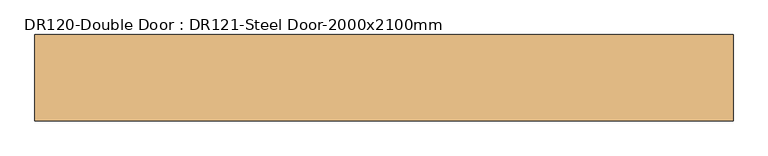
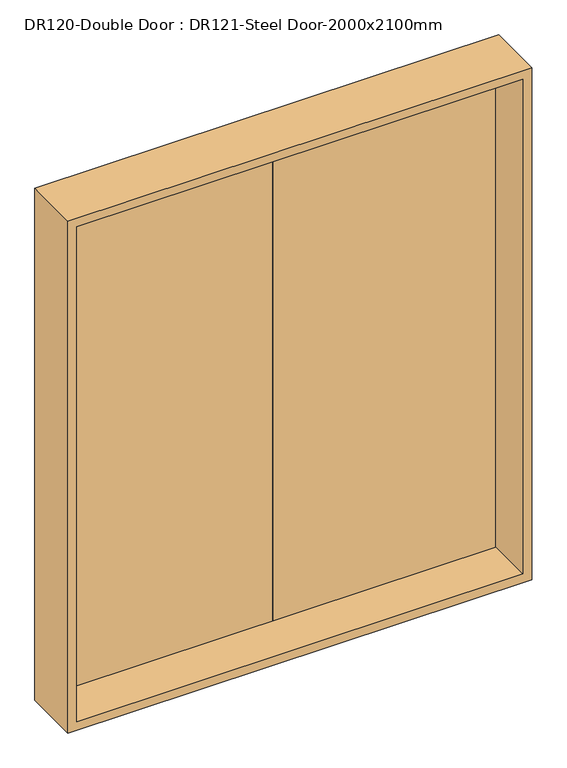
"""IFC4 building model written with IfcOpenShell, lengths in millimetres: door geometry, DR120-Double Door : DR121-Steel Door-2000x2100mm."""

from ifc_helpers import new_model, si_unit, frame, origin, place, context, project, spatial, polyline, outline, extrude, faceted_brep, source, transform, mapped, element, save


def dr120_double_door_dr121_steel_door_2000x2100mm_bb3c48ff(model_context):
    return source(origin(), model_context, "Body", "SolidModel", [
        extrude(outline(polyline([(880.0, 71.0), (0.0, 71.0), (0.0, 111.0), (880.0, 111.0), (880.0, 71.0)])), frame((0.0, 0.0, 20.0), z_axis=(0.0, 0.0, 1.0), x_axis=(1.0, 0.0, 0.0)), (0.0, 0.0, 1.0), 2060.0),
        extrude(outline(polyline([(0.0, 71.0), (-880.0, 71.0), (-880.0, 111.0), (0.0, 111.0), (0.0, 71.0)])), frame((0.0, 0.0, 20.0), z_axis=(0.0, 0.0, 1.0), x_axis=(1.0, 0.0, 0.0)), (0.0, 0.0, 1.0), 2060.0),
        faceted_brep([(900.0, -111.0, 2100.0), (900.0, 111.0, 2100.0), (-900.0, 111.0, 2100.0), (-900.0, -111.0, 2100.0), (865.0, 71.0, 2065.0), (865.0, -111.0, 2065.0), (-865.0, -111.0, 2065.0), (-865.0, 71.0, 2065.0), (880.0, 111.0, 2080.0), (880.0, 71.0, 2080.0), (-880.0, 71.0, 2080.0), (-880.0, 111.0, 2080.0), (-900.0, 111.0, 0.0), (-900.0, -111.0, 0.0), (-865.0, -111.0, 35.0), (-865.0, 71.0, 35.0), (-880.0, 71.0, 20.0), (-880.0, 111.0, 20.0), (900.0, 111.0, 0.0), (880.0, 111.0, 20.0), (900.0, -111.0, 0.0), (865.0, -111.0, 35.0), (865.0, 71.0, 35.0), (880.0, 71.0, 20.0)], [[[0, 1, 2, 3]], [[4, 5, 6, 7]], [[8, 9, 10, 11]], [[3, 2, 12, 13]], [[7, 6, 14, 15]], [[11, 10, 16, 17]], [[18, 12, 2, 1], [8, 11, 17, 19]], [[13, 12, 18, 20]], [[0, 3, 13, 20], [21, 14, 6, 5]], [[15, 14, 21, 22]], [[23, 16, 10, 9], [4, 7, 15, 22]], [[17, 16, 23, 19]], [[20, 18, 1, 0]], [[22, 21, 5, 4]], [[19, 23, 9, 8]]]),
    ])


if __name__ == "__main__":
    model = new_model("IFC4")
    model_context = context("Model", 3, world=origin())
    ifc_project = project(units=[si_unit("LENGTHUNIT", "METRE", prefix="MILLI")], contexts=[model_context])
    site = spatial("IfcSite", under=ifc_project)
    building = spatial("IfcBuilding", under=site)
    placement = place(None, origin())
    dr120_double_door_dr121_steel_door_2000x2100mm_shape = dr120_double_door_dr121_steel_door_2000x2100mm_bb3c48ff(model_context)
    element("IfcDoor", 1, ObjectType="DR120-Double Door : DR121-Steel Door-2000x2100mm", at=placement, inside=building, context=model_context, shape_type="MappedRepresentation", body=[
        mapped(dr120_double_door_dr121_steel_door_2000x2100mm_shape, transform((0.0, 0.0, 0.0), x_axis=(1.0, 0.0, 0.0), y_axis=(0.0, 1.0, 0.0), z_axis=(0.0, 0.0, 1.0))),
    ])
    save(model, "model.ifc")

# Revit data of these elements
# Type "DR120-Double Door : DR121-Steel Door-2000x2100mm"
#   Type Mark = "SD"
#   프레임 = ""
#   철물 = ""
#   유리/마감 = ""
#   위치/개소 = ""
#   부호 = "1/SD"
#   문번호 = ""
#   문기호 = "SD"
#   Analytic Construction = "<None>"
#   Height = 2100 mm
#   Width = 1800 mm
#   Define Thermal Properties by = 1
#   문 틀 = A04AQ098-00003_Steel Door_non FP_double
#   문 = 문
#   Function = (empty or 0)
#   Assembly Code = ""
#   Wall Closure = (empty or 0)
# Element 1 (IfcDoor, "DR120-Double Door : DR121-Steel Door-2000x2100mm")
#   Materials on its faces: "A04AQ098-00003_Steel Door_non FP_double", "문"
# Materials
#   "A04AQ098-00003_Steel Door_non FP_double": class "금속", colour RGB 247 247 247, transparency 0, Description = "Steel Door", W00) Work Master Code = "A04AQ098-00003", W01) Work Master_Lv1 = "Finishing Work", W02) Work Master_Lv2 = "Door & Window Work", W03) Work Master_Spec.1 = "Steel Door w/ Steel Frame", W04) Work Master_Spec.2 = "Fire Protective Rating: N/A, Double Door", W05) Work Master_Spec.3 = "w/ Hardware & Accessories", Cost = 0
#   "문": class "다양한", colour RGB 247 247 247, transparency 0
